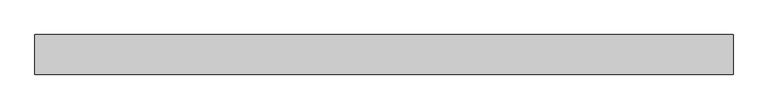
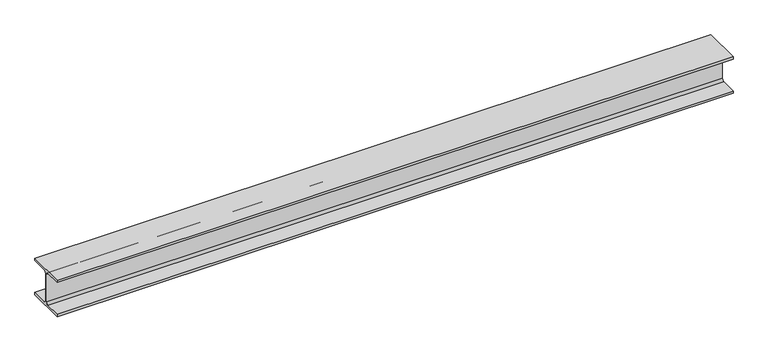
"""IFC4 building model written with IfcOpenShell, lengths in millimetres: beam geometry, 0912_Steel Framing_H-KSD3502 : H_SB_ASB_H-200x200x8x12."""

from ifc_helpers import new_model, si_unit, point, frame, frame_2d, origin, place, context, project, spatial, polyline, circle_curve, trimmed, segment, composite_curve, outline, extrude, source, transform, mapped, element, save


def beam_be79e5d0(model_context):
    return source(origin(), model_context, "Body", "SweptSolid", [
        extrude(outline(composite_curve([segment(polyline([(100.0, -88.0), (100.0, -100.0), (-100.0, -100.0), (-100.0, -88.0), (-17.0, -88.0)]), True, "CONTINUOUS"), segment(trimmed(circle_curve(frame_2d((-17.0, -75.0)), 13.0), [point((-17.0, -88.0))], [point((-4.0, -75.0))], True, "CARTESIAN"), True, "CONTINUOUS"), segment(polyline([(-4.0, -75.0), (-4.0, 75.0)]), True, "CONTINUOUS"), segment(trimmed(circle_curve(frame_2d((-17.0, 75.0)), 13.0), [point((-4.0, 75.0))], [point((-17.0, 88.0))], True, "CARTESIAN"), True, "CONTINUOUS"), segment(polyline([(-17.0, 88.0), (-100.0, 88.0), (-100.0, 100.0), (100.0, 100.0), (100.0, 88.0), (17.0, 88.0)]), True, "CONTINUOUS"), segment(trimmed(circle_curve(frame_2d((17.0, 75.0)), 13.0), [point((17.0, 88.0))], [point((4.0, 75.0))], True, "CARTESIAN"), True, "CONTINUOUS"), segment(polyline([(4.0, 75.0), (4.0, -75.0)]), True, "CONTINUOUS"), segment(trimmed(circle_curve(frame_2d((17.0, -75.0)), 13.0), [point((4.0, -75.0))], [point((17.0, -88.0))], True, "CARTESIAN"), True, "CONTINUOUS"), segment(polyline([(17.0, -88.0), (100.0, -88.0)]), True, "CONTINUOUS")], self_intersect=False)), frame((-1810.5748531, 0.0, 0.0), z_axis=(1.0, 0.0, 0.0), x_axis=(0.0, 1.0, 0.0)), (0.0, 0.0, 1.0), 3520.5189629),
    ])


if __name__ == "__main__":
    model = new_model("IFC4")
    model_context = context("Model", 3, world=origin())
    ifc_project = project(units=[si_unit("LENGTHUNIT", "METRE", prefix="MILLI")], contexts=[model_context])
    site = spatial("IfcSite", under=ifc_project)
    building = spatial("IfcBuilding", under=site)
    placement = place(None, origin())
    beam_shape = beam_be79e5d0(model_context)
    element("IfcBeam", 1, ObjectType="0912_Steel Framing_H-KSD3502 : H_SB_ASB_H-200x200x8x12", at=placement, inside=building, context=model_context, shape_type="MappedRepresentation", body=[
        mapped(beam_shape, transform((0.0, 0.0, 0.0), x_axis=(1.0, 0.0, 0.0), y_axis=(0.0, 1.0, 0.0), z_axis=(0.0, 0.0, 1.0))),
    ])
    save(model, "model.ifc")

# Revit data of these elements
# Type "0912_Steel Framing_H-KSD3502 : H_SB_ASB_H-200x200x8x12"
#   H_WM Code_1 = "S01AA002-00001 | Main Steel Structure Fabrication Work | Shelter/Building | Medium Steel - Standard (90KG/M>Weight≥30KG/M) | Material: (   )"
#   H_WM Code_2 = "S03AA028-00001 | Main Steel Structure Erection Work | Shelter/Building | Medium Steel (90KG/M>Weight≥30KG/M) | Material: (   )"
#   H_WM Code_3 = "S01AA010-00001 | Main Steel Structure Fabrication Work | Shelter/Building | Steel Painting/Coating | for Non-Fireproofed Steel Surface, Surface Preparation, Primer, Second & Final Coat | Material: (   )"
#   H_Q'ty Cal Type Tag = "SB-Q2"
#   Width = 20.0 cm
#   Web Thickness = 0.8 cm
#   Web Fillet = 1.3 cm
#   Warping Constant = 141000.0 cm⁶
#   W = 0
#   Torsional Moment of Inertia = 26.2485 cm⁴
#   Section Area = 63.53 cm²
#   Plastic Modulus weak axis = 244.0 cm³
#   Plastic Modulus strong axis = 525.0 cm³
#   Perimeter = 1.16 m²/m
#   Nominal Weight = 49.90 kgf/m
#   Moment of Inertia weak axis = 1600.00 cm⁴
#   Moment of Inertia strong axis = 4720.00 cm⁴
#   Height = 20.0 cm
#   Flange Thickness = 1.2 cm
#   Elastic Modulus weak axis = 160.0 cm³
#   Elastic Modulus strong axis = 472.0 cm³
#   Centroid Vertical = 10.0 cm
#   Centroid Horizontal = 10.0 cm
#   Ix = 47200000
#   Length [instance default] = 1.5240 m
#   Zx = 525000
#   b = 0.2000 m
#   h = 0.2000 m
#   r = 0.0130 m
#   s = 0.0080 m
#   t = 0.0120 m
#   A = 0.006353 m²
#   Structural Material [instance default] = Steel, 45-345
#   Assembly Code = ""
# Element 1 (IfcBeam, "0912_Steel Framing_H-KSD3502 : H_SB_ASB_H-200x200x8x12")
#   Structural Material = none
# Materials
#   "Steel, 45-345": class "Metal", colour RGB 189 187 185, transparency 0, Description = "Steel 345 MPa", Cost = 0
